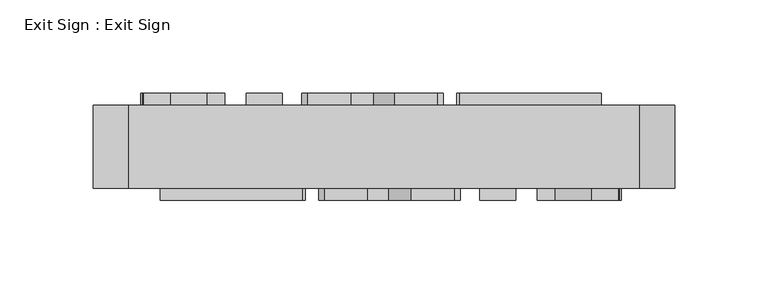
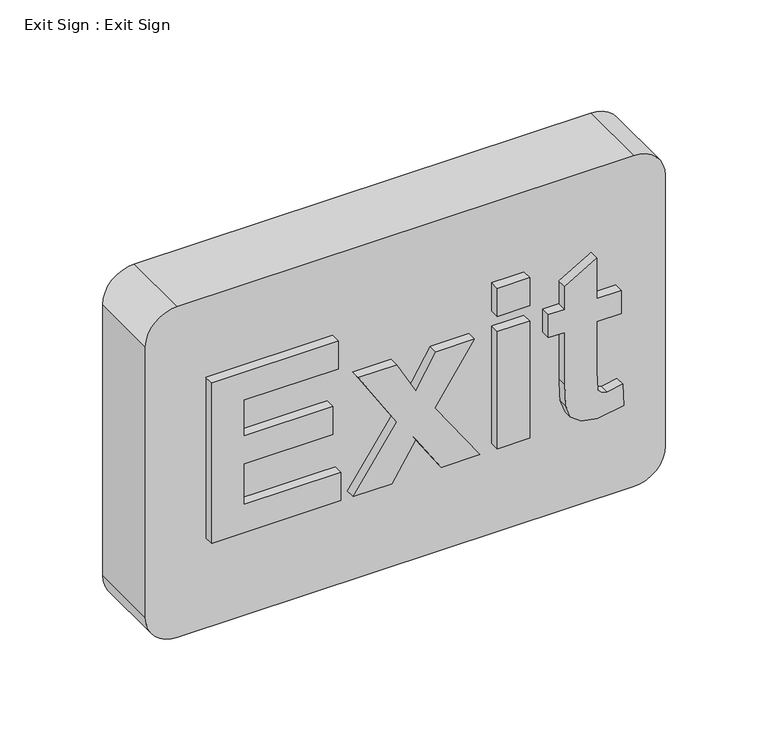
"""IFC4 building model written with IfcOpenShell, lengths in millimetres: proxy geometry, Exit Sign : Exit Sign."""

import ifcopenshell
import ifcopenshell.guid

model = None  # the IFC model being written
_history = None  # IfcOwnerHistory: only IFC2X3 demands one
_inside = {}  # id of a spatial element -> (the spatial element, [elements in it])
_under = {}  # id of a project, library or spatial element -> (it, [spatial elements below it])
_declared = {}  # id of a project -> (the project, [libraries it declares])
_typed = {}  # id of a type object -> (the type object, [elements of that type])
_made_of = {}  # id of a material, layer set ... -> (it, [elements and type objects made of it])


def new_model(schema):
    """Start an empty IFC model of exactly this schema.

    Asked for "IFC4X3", IfcOpenShell would pick the latest addendum, in which some entities
    have other attributes; the version numbers below select the first issue.
    IFC2X3 requires an IfcOwnerHistory on every rooted entity: one is made here for all.
    """
    global model, _history
    if schema == "IFC4X3":
        model = ifcopenshell.file(schema_version=(4, 3, 0, 0))
    else:
        model = ifcopenshell.file(schema=schema)
    _inside.clear()
    _under.clear()
    _declared.clear()
    _typed.clear()
    _made_of.clear()
    _history = None
    if model.schema == "IFC2X3":
        org = make("IfcOrganization", Name="unknown")
        user = make(
            "IfcPersonAndOrganization",
            ThePerson=make("IfcPerson", FamilyName="unknown"),
            TheOrganization=org,
        )
        app = make(
            "IfcApplication",
            ApplicationDeveloper=org,
            Version="unknown",
            ApplicationFullName="unknown",
            ApplicationIdentifier="unknown",
        )
        _history = make(
            "IfcOwnerHistory",
            OwningUser=user,
            OwningApplication=app,
            ChangeAction="ADDED",
            CreationDate=0,
        )
    return model


def make(cls, **values):
    """One entity of the class cls with the attributes given. An attribute that is None is left unset."""
    return model.create_entity(
        cls, **{name: value for name, value in values.items() if value is not None}
    )


def rooted(cls, **values):
    """An entity with a GlobalId (a new one), such as an element, a storey or a relation."""
    return make(cls, GlobalId=ifcopenshell.guid.new(), OwnerHistory=_history, **values)


def si_unit(unit_type, name, prefix=None):
    """IfcSIUnit, for example si_unit("LENGTHUNIT", "METRE", prefix="MILLI")."""
    return make("IfcSIUnit", UnitType=unit_type, Prefix=prefix, Name=name)


def assignment(units):
    """IfcUnitAssignment: the units of a project."""
    return None if units is None else make("IfcUnitAssignment", Units=units)


def point(xyz):
    """IfcCartesianPoint."""
    return None if xyz is None else make("IfcCartesianPoint", Coordinates=xyz)


def direction(xyz):
    """IfcDirection."""
    return None if xyz is None else make("IfcDirection", DirectionRatios=xyz)


def frame(location, z_axis=None, x_axis=None):
    """IfcAxis2Placement3D, a coordinate frame: its origin and axes. An axis left out is left unset."""
    return make(
        "IfcAxis2Placement3D",
        Location=point(location),
        Axis=direction(z_axis),
        RefDirection=direction(x_axis),
    )


def frame_2d(location, x_axis=None):
    """IfcAxis2Placement2D, a coordinate frame in the plane: its origin and x axis."""
    return make(
        "IfcAxis2Placement2D", Location=point(location), RefDirection=direction(x_axis)
    )


def origin():
    """The frame at (0, 0, 0) with its axes left unset."""
    return frame((0.0, 0.0, 0.0))


def place(relative_to, where):
    """IfcLocalPlacement: puts the frame where relative to a parent placement (None: the world)."""
    return make(
        "IfcLocalPlacement", PlacementRelTo=relative_to, RelativePlacement=where
    )


def context(
    kind, dimensions, precision=None, world=None, true_north=None, identifier=None
):
    """IfcGeometricRepresentationContext, for example the 3D "Model" context."""
    return make(
        "IfcGeometricRepresentationContext",
        ContextIdentifier=identifier,
        ContextType=kind,
        CoordinateSpaceDimension=dimensions,
        Precision=precision,
        WorldCoordinateSystem=world,
        TrueNorth=true_north,
    )


def project(units=None, contexts=None):
    """IfcProject with its units and contexts."""
    return rooted(
        "IfcProject",
        Name="project",
        RepresentationContexts=contexts,
        UnitsInContext=assignment(units),
    )


def spatial(cls, under=None, at=None, **own):
    """A site, building, storey or space (cls), placed at a placement, below another one or the project."""
    s = rooted(cls, ObjectPlacement=at, **own)
    if under is not None:
        _under.setdefault(under.id(), (under, []))[1].append(s)
    return s


def polyline(points):
    """IfcPolyline through the points."""
    return make("IfcPolyline", Points=[point(p) for p in points])


def circle_curve(where, radius):
    """IfcCircle in the frame where."""
    return make("IfcCircle", Position=where, Radius=radius)


def trimmed(basis, trim1, trim2, sense, master):
    """IfcTrimmedCurve: the piece of a basis curve between two trims."""
    return make(
        "IfcTrimmedCurve",
        BasisCurve=basis,
        Trim1=trim1,
        Trim2=trim2,
        SenseAgreement=sense,
        MasterRepresentation=master,
    )


def segment(curve, same_sense, transition):
    """IfcCompositeCurveSegment."""
    return make(
        "IfcCompositeCurveSegment",
        Transition=transition,
        SameSense=same_sense,
        ParentCurve=curve,
    )


def composite_curve(segments, self_intersect=None):
    """IfcCompositeCurve: segments joined end to end."""
    return make("IfcCompositeCurve", Segments=segments, SelfIntersect=self_intersect)


def outline(outer, holes=None, kind="AREA"):
    """IfcArbitraryClosedProfileDef: a profile drawn as a closed curve; with holes, ...WithVoids."""
    if holes is None:
        return make("IfcArbitraryClosedProfileDef", ProfileType=kind, OuterCurve=outer)
    return make(
        "IfcArbitraryProfileDefWithVoids",
        ProfileType=kind,
        OuterCurve=outer,
        InnerCurves=holes,
    )


def extrude(swept, where, along, depth):
    """IfcExtrudedAreaSolid: the profile swept, set in the frame where, extruded along a direction by depth."""
    return make(
        "IfcExtrudedAreaSolid",
        SweptArea=swept,
        Position=where,
        ExtrudedDirection=direction(along),
        Depth=depth,
    )


def shape(context_of_items, identifier, shape_type, items):
    """IfcShapeRepresentation: the items that make up one representation, for example the "Body"."""
    return make(
        "IfcShapeRepresentation",
        ContextOfItems=context_of_items,
        RepresentationIdentifier=identifier,
        RepresentationType=shape_type,
        Items=items,
    )


def source(mapping_origin, context_of_items, identifier, shape_type, items):
    """IfcRepresentationMap: a shape defined once, which mapped items show again and again."""
    return make(
        "IfcRepresentationMap",
        MappingOrigin=mapping_origin,
        MappedRepresentation=shape(context_of_items, identifier, shape_type, items),
    )


def transform(
    local_origin,
    x_axis=None,
    y_axis=None,
    z_axis=None,
    scale=None,
    scale2=None,
    scale3=None,
    uniform=True,
):
    """IfcCartesianTransformationOperator3D, or its non-uniform kind. x_axis, y_axis, z_axis: its Axis1, 2, 3."""
    if uniform:
        return make(
            "IfcCartesianTransformationOperator3D",
            Axis1=direction(x_axis),
            Axis2=direction(y_axis),
            LocalOrigin=point(local_origin),
            Scale=scale,
            Axis3=direction(z_axis),
        )
    return make(
        "IfcCartesianTransformationOperator3DnonUniform",
        Axis1=direction(x_axis),
        Axis2=direction(y_axis),
        LocalOrigin=point(local_origin),
        Scale=scale,
        Axis3=direction(z_axis),
        Scale2=scale2,
        Scale3=scale3,
    )


def mapped(mapping_source, mapping_target):
    """IfcMappedItem: shows the shape of a source again, moved by a transform."""
    return make(
        "IfcMappedItem", MappingSource=mapping_source, MappingTarget=mapping_target
    )


def made_of(thing, what):
    """Note that an element or type object is made of a material, layer set ...; save() writes the relation."""
    if what is not None:
        _made_of.setdefault(what.id(), (what, []))[1].append(thing)
    return thing


def element(
    cls,
    number,
    at=None,
    inside=None,
    cuts=None,
    type_object=None,
    material=None,
    context=None,
    identifier="Body",
    shape_type=None,
    held_by="IfcProductDefinitionShape",
    body=None,
    shapes=None,
    **own,
):
    """One element of the class cls, such as IfcWall. Its Tag is "e" and its number.

    at: its placement. inside: the storey or other place that contains it. cuts: it is an
    opening in that element (IfcRelVoidsElement). A single representation is given by context,
    identifier, shape_type and body (its items); several are given by shapes. held_by: the class
    of the entity that holds the representations. save() writes the other relations.
    """
    e = rooted(cls, Tag="e%d" % number, ObjectPlacement=at, **own)
    if body is not None:
        shapes = [shape(context, identifier, shape_type, body)]
    if shapes is not None:
        e.Representation = make(held_by, Representations=shapes)
    if inside is not None:
        _inside.setdefault(inside.id(), (inside, []))[1].append(e)
    if cuts is not None:
        rooted(
            "IfcRelVoidsElement", RelatingBuildingElement=cuts, RelatedOpeningElement=e
        )
    if type_object is not None:
        _typed.setdefault(type_object.id(), (type_object, []))[1].append(e)
    return made_of(e, material)


def aggregate(whole, parts):
    """IfcRelAggregates: a whole, such as a stair, and the parts it consists of."""
    return rooted("IfcRelAggregates", RelatingObject=whole, RelatedObjects=parts)


def save(model, path):
    """Write the relations noted so far, then the file.

    IfcRelAggregates (storeys below a building ...), IfcRelContainedInSpatialStructure (elements
    in a storey), IfcRelDefinesByType, IfcRelAssociatesMaterial and IfcRelDeclares: one each for
    every whole, place, type object, material and project.
    """
    for whole, parts in _under.values():
        aggregate(whole, parts)
    for where, things in _inside.values():
        rooted(
            "IfcRelContainedInSpatialStructure",
            RelatedElements=things,
            RelatingStructure=where,
        )
    for kind, things in _typed.values():
        rooted("IfcRelDefinesByType", RelatedObjects=things, RelatingType=kind)
    for what, things in _made_of.values():
        rooted("IfcRelAssociatesMaterial", RelatedObjects=things, RelatingMaterial=what)
    for by, libraries in _declared.values():
        rooted("IfcRelDeclares", RelatingContext=by, RelatedDefinitions=libraries)
    model.write(path)


def exit_sign_exit_sign_daf696ad(model_context):
    return source(origin(), model_context, "Body", "SweptSolid", [
        extrude(outline(composite_curve([segment(polyline([(2438.4, 136.525), (2438.4, -136.525)]), True, "CONTINUOUS"), segment(trimmed(circle_curve(frame_2d((2419.35, -136.525)), 19.05), [point((2438.4, -136.525))], [point((2419.35, -155.575))], False, "CARTESIAN"), True, "CONTINUOUS"), segment(polyline([(2419.35, -155.575), (2247.9, -155.575)]), True, "CONTINUOUS"), segment(trimmed(circle_curve(frame_2d((2247.9, -136.525)), 19.05), [point((2247.9, -155.575))], [point((2228.85, -136.525))], False, "CARTESIAN"), True, "CONTINUOUS"), segment(polyline([(2228.85, -136.525), (2228.85, 136.525)]), True, "CONTINUOUS"), segment(trimmed(circle_curve(frame_2d((2247.9, 136.525)), 19.05), [point((2228.85, 136.525))], [point((2247.9, 155.575))], False, "CARTESIAN"), True, "CONTINUOUS"), segment(polyline([(2247.9, 155.575), (2419.35, 155.575)]), True, "CONTINUOUS"), segment(trimmed(circle_curve(frame_2d((2419.35, 136.525)), 19.05), [point((2419.35, 155.575))], [point((2438.4, 136.525))], False, "CARTESIAN"), True, "CONTINUOUS")], self_intersect=False)), frame((0.0, -34.925, 0.0), z_axis=(0.0, 1.0, 0.0), x_axis=(0.0, 0.0, 1.0)), (0.0, 0.0, 1.0), 44.45),
        extrude(outline(polyline([(2286.4280581, -119.6667099), (2286.4280581, -42.2571861), (2304.1677406, -42.2571861), (2304.1677406, -100.314329), (2329.9709152, -100.314329), (2329.9709152, -47.0952813), (2347.7105977, -47.0952813), (2347.7105977, -100.314329), (2370.2883755, -100.314329), (2370.2883755, -43.8698845), (2388.0280581, -43.8698845), (2388.0280581, -119.6667099), (2286.4280581, -119.6667099)])), frame((0.0, -41.275, 0.0), z_axis=(0.0, 1.0, 0.0), x_axis=(0.0, 0.0, 1.0)), (0.0, 0.0, 1.0), 6.35),
        extrude(outline(polyline([(2286.4280581, -35.0000432), (2286.4280581, -11.9938925), (2309.4090104, 2.4195996), (2286.4280581, 17.7906314), (2286.4280581, 40.7967822), (2325.4855977, 13.9100758), (2360.612185, 37.5713853), (2360.612185, 14.5652345), (2340.2266692, 2.4195996), (2360.612185, -8.7684956), (2360.612185, -31.7746464), (2324.6288517, -8.793694), (2286.4280581, -35.0000432)])), frame((0.0, -41.275, 0.0), z_axis=(0.0, 1.0, 0.0), x_axis=(0.0, 0.0, 1.0)), (0.0, 0.0, 1.0), 6.35),
        extrude(outline(polyline([(70.6317028, -41.275), (51.2793218, -41.275), (51.2793218, -34.925), (70.6317028, -34.925), (70.6317028, -41.275)])), frame((0.0, 0.0, 2370.2883755), z_axis=(0.0, 0.0, 1.0), x_axis=(1.0, 0.0, 0.0)), (0.0, 0.0, 1.0), 17.7396825),
        extrude(outline(polyline([(70.6317028, -41.275), (51.2793218, -41.275), (51.2793218, -34.925), (70.6317028, -34.925), (70.6317028, -41.275)])), frame((0.0, 0.0, 2286.4280581), z_axis=(0.0, 0.0, 1.0), x_axis=(1.0, 0.0, 0.0)), (0.0, 0.0, 1.0), 74.184127),
        extrude(outline(polyline([(2360.612185, 125.4634488), (2360.612185, 110.9491631), (2386.4153597, 110.9491631), (2375.1264708, 91.5967822), (2360.612185, 91.5967822), (2360.612185, 81.9205917), (2346.0978993, 81.9205917), (2346.0978993, 91.5967822), (2313.1887723, 91.5967822), (2299.1028597, 92.2267425), (2291.3165501, 95.0615639), (2286.6296454, 101.4493615), (2284.8153597, 111.2263456), (2287.4359946, 127.0761472), (2301.1943279, 126.269798), (2299.3296454, 117.1983695), (2300.3753795, 113.3934091), (2303.0212128, 111.3901353), (2314.2723041, 110.9491631), (2346.0978993, 110.9491631), (2346.0978993, 125.4634488), (2360.612185, 125.4634488)])), frame((0.0, -41.275, 0.0), z_axis=(0.0, 1.0, 0.0), x_axis=(0.0, 0.0, 1.0)), (0.0, 0.0, 1.0), 6.35),
        extrude(outline(polyline([(2284.0985242, 116.4382316), (2385.6985242, 116.4382316), (2385.6985242, 40.6414062), (2367.9588417, 40.6414062), (2367.9588417, 97.0858507), (2345.3810639, 97.0858507), (2345.3810639, 43.866803), (2327.6413814, 43.866803), (2327.6413814, 97.0858507), (2301.8382068, 97.0858507), (2301.8382068, 39.0287078), (2284.0985242, 39.0287078), (2284.0985242, 116.4382316)])), frame((0.0, 9.525, 0.0), z_axis=(0.0, 1.0, 0.0), x_axis=(0.0, 0.0, 1.0)), (0.0, 0.0, 1.0), 6.35),
        extrude(outline(polyline([(2284.0985242, 31.7715649), (2322.2993179, 5.5652157), (2358.2826512, 28.5461681), (2358.2826512, 5.5400173), (2337.8971354, -5.6480779), (2358.2826512, -17.7937128), (2358.2826512, -40.7998636), (2323.1560639, -17.1385541), (2284.0985242, -44.0252605), (2284.0985242, -21.0191097), (2307.0794766, -5.6480779), (2284.0985242, 8.7654141), (2284.0985242, 31.7715649)])), frame((0.0, 9.525, 0.0), z_axis=(0.0, 1.0, 0.0), x_axis=(0.0, 0.0, 1.0)), (0.0, 0.0, 1.0), 6.35),
        extrude(outline(polyline([(-73.8601811, 15.875), (-54.5078001, 15.875), (-54.5078001, 9.525), (-73.8601811, 9.525), (-73.8601811, 15.875)])), frame((0.0, 0.0, 2367.9588417), z_axis=(0.0, 0.0, 1.0), x_axis=(1.0, 0.0, 0.0)), (0.0, 0.0, 1.0), 17.7396825),
        extrude(outline(polyline([(-73.8601811, 15.875), (-54.5078001, 15.875), (-54.5078001, 9.525), (-73.8601811, 9.525), (-73.8601811, 15.875)])), frame((0.0, 0.0, 2284.0985242), z_axis=(0.0, 0.0, 1.0), x_axis=(1.0, 0.0, 0.0)), (0.0, 0.0, 1.0), 74.184127),
        extrude(outline(polyline([(2358.2826512, -128.6919271), (2343.7683655, -128.6919271), (2343.7683655, -114.1776414), (2311.9427703, -114.1776414), (2300.691679, -114.6186136), (2298.0458457, -116.6218874), (2297.0001115, -120.4268478), (2298.8647941, -129.4982763), (2285.1064607, -130.3046255), (2282.4858258, -114.4548239), (2284.3001115, -104.6778398), (2288.9870163, -98.2900422), (2296.7733258, -95.4552208), (2310.8592385, -94.8252605), (2343.7683655, -94.8252605), (2343.7683655, -85.14907), (2358.2826512, -85.14907), (2358.2826512, -94.8252605), (2372.7969369, -94.8252605), (2384.0858258, -114.1776414), (2358.2826512, -114.1776414), (2358.2826512, -128.6919271)])), frame((0.0, 9.525, 0.0), z_axis=(0.0, 1.0, 0.0), x_axis=(0.0, 0.0, 1.0)), (0.0, 0.0, 1.0), 6.35),
    ])


if __name__ == "__main__":
    model = new_model("IFC4")
    model_context = context("Model", 3, world=origin())
    ifc_project = project(units=[si_unit("LENGTHUNIT", "METRE", prefix="MILLI")], contexts=[model_context])
    site = spatial("IfcSite", under=ifc_project)
    building = spatial("IfcBuilding", under=site)
    placement = place(None, origin())
    exit_sign_exit_sign_shape = exit_sign_exit_sign_daf696ad(model_context)
    element("IfcBuildingElementProxy", 1, Name="Exit Sign : Exit Sign", ObjectType="Exit Sign : Exit Sign", at=placement, inside=building, context=model_context, shape_type="MappedRepresentation", body=[
        mapped(exit_sign_exit_sign_shape, transform((0.0, 0.0, 0.0), x_axis=(1.0, 0.0, 0.0), y_axis=(0.0, 1.0, 0.0), z_axis=(0.0, 0.0, 1.0))),
    ])
    save(model, "model.ifc")

# Revit data of these elements
# Type "Exit Sign : Exit Sign"
#   Assembly Code = "D5090200"
#   Default Elevation = 0
# Element 1 (IfcBuildingElementProxy, "Exit Sign : Exit Sign")
#   Materials on its faces: "Red Lettering", "Steel, Paint Finish, Ivory, Glossy"
# Materials
#   "Red Lettering": class "Miscellaneous", colour RGB 200 0 0, transparency 0
#   "Steel, Paint Finish, Ivory, Glossy": class "Metal", colour RGB 247 247 239, transparency 0, Description = "Steel, paint finish, ivory, glossy", Cost = 0
